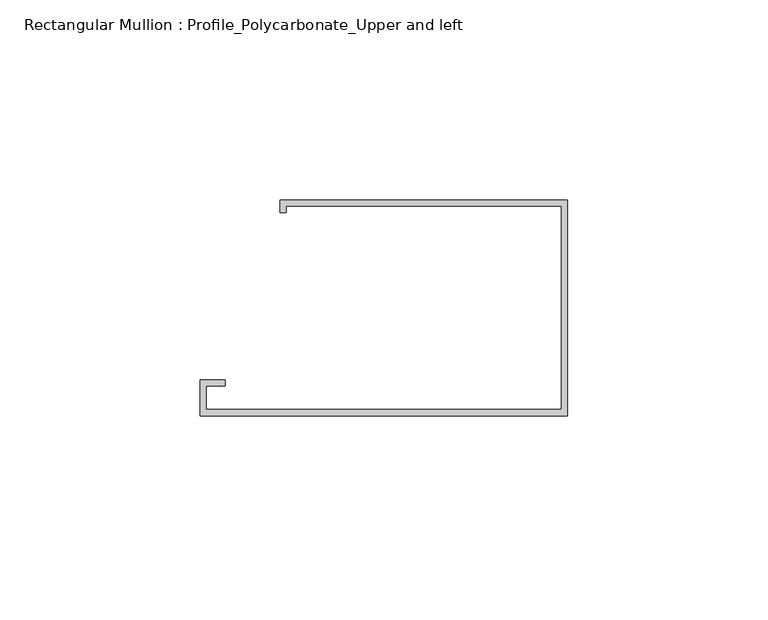
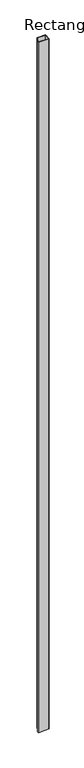
"""IFC4 building model written with IfcOpenShell, lengths in millimetres: member geometry, Rectangular Mullion : Profile_Polycarbonate_Upper and left."""

from ifc_helpers import new_model, si_unit, frame, origin, place, context, project, spatial, polyline, outline, extrude, source, transform, mapped, element, save


def rectangular_mullion_profile_polycarbonate_upper_and_left_6d5b298c(model_context):
    return source(origin(), model_context, "Body", "SweptSolid", [
        extrude(outline(polyline([(0.0, -28.984575), (-91.9988, -28.984575), (-91.9988, -19.992975), (-85.6488, -19.992975), (-85.6488, -21.580475), (-90.4113, -21.580475), (-90.4113, -27.397075), (-1.5875, -27.397075), (-1.5875, 23.428325), (-70.3961, 23.428325), (-70.3961, 21.840825), (-71.9836, 21.840825), (-71.9836, 25.015825), (0.0, 25.015825), (0.0, -28.984575)])), frame((0.0, 0.0, -6191.0976), z_axis=(0.0, 0.0, 1.0), x_axis=(1.0, 0.0, 0.0)), (0.0, 0.0, 1.0), 6191.0976),
    ])


if __name__ == "__main__":
    model = new_model("IFC4")
    model_context = context("Model", 3, world=origin())
    ifc_project = project(units=[si_unit("LENGTHUNIT", "METRE", prefix="MILLI")], contexts=[model_context])
    site = spatial("IfcSite", under=ifc_project)
    building = spatial("IfcBuilding", under=site)
    placement = place(None, origin())
    rectangular_mullion_profile_polycarbonate_upper_and_left_shape = rectangular_mullion_profile_polycarbonate_upper_and_left_6d5b298c(model_context)
    element("IfcMember", 1, ObjectType="Rectangular Mullion : Profile_Polycarbonate_Upper and left", at=placement, inside=building, context=model_context, shape_type="MappedRepresentation", body=[
        mapped(rectangular_mullion_profile_polycarbonate_upper_and_left_shape, transform((0.0, 0.0, 0.0), x_axis=(1.0, 0.0, 0.0), y_axis=(0.0, 1.0, 0.0), z_axis=(0.0, 0.0, 1.0))),
    ])
    save(model, "model.ifc")

# Revit data of these elements
# Type "Rectangular Mullion : Profile_Polycarbonate_Upper and left"
#   built-in parameter 1007322 = 0.177167 (stored number, unit not read)
#   built-in parameter 1007321 = 0.00520833 (stored number, unit not read)
#   built-in parameter 1007320 = 0 (stored number, unit not read)
